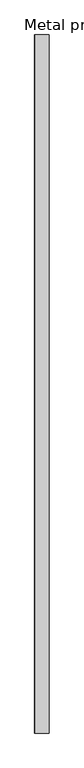
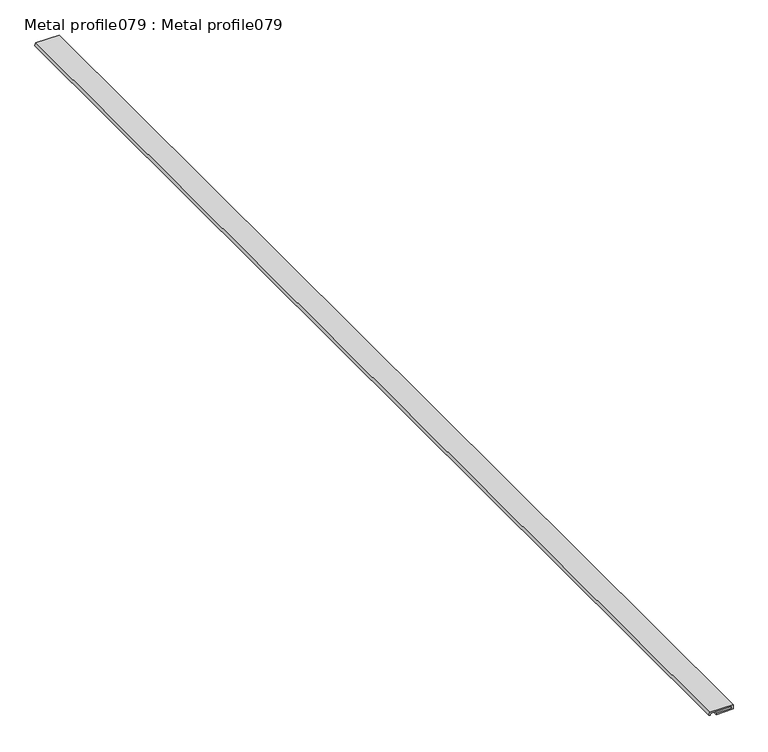
"""IFC4 building model written with IfcOpenShell, lengths in millimetres: proxy geometry, Metal profile079 : Metal profile079."""

from ifc_helpers import new_model, si_unit, frame, origin, place, context, project, spatial, polyline, outline, extrude, source, transform, mapped, element, save


def metal_profile079_metal_profile079_eafd9208(model_context):
    return source(origin(), model_context, "Body", "SweptSolid", [
        extrude(outline(polyline([(40172.6132812, -9397.2722564), (40170.6132812, -9397.2722564), (40170.6132812, -9368.0046783), (40177.890625, -9368.0046783), (40178.484375, -9407.6785064), (40173.4296875, -9409.304483), (40172.8172405, -9407.4005637), (40176.4624429, -9406.227986), (40175.9203326, -9370.0046783), (40172.6132812, -9370.0046783), (40172.6132812, -9397.2722564)])), frame((0.0, 7982.1531721, 0.0), z_axis=(0.0, 1.0, 0.0), x_axis=(0.0, 0.0, 1.0)), (0.0, 0.0, 1.0), 2000.0),
    ])


if __name__ == "__main__":
    model = new_model("IFC4")
    model_context = context("Model", 3, world=origin())
    ifc_project = project(units=[si_unit("LENGTHUNIT", "METRE", prefix="MILLI")], contexts=[model_context])
    site = spatial("IfcSite", under=ifc_project)
    building = spatial("IfcBuilding", under=site)
    placement = place(None, origin())
    metal_profile079_metal_profile079_shape = metal_profile079_metal_profile079_eafd9208(model_context)
    element("IfcBuildingElementProxy", 1, Name="Metal profile079 : Metal profile079", ObjectType="Metal profile079 : Metal profile079", at=placement, inside=building, context=model_context, shape_type="MappedRepresentation", body=[
        mapped(metal_profile079_metal_profile079_shape, transform((0.0, 0.0, 0.0), x_axis=(1.0, 0.0, 0.0), y_axis=(0.0, 1.0, 0.0), z_axis=(0.0, 0.0, 1.0))),
    ])
    save(model, "model.ifc")

# Revit data of these elements
# Type "Metal profile079 : Metal profile079"
#   NameOverride = "Metal profile079"
# Element 1 (IfcBuildingElementProxy, "Metal profile079 : Metal profile079")
#   Materials on its faces: "ANGLE TRIM"
# Materials
#   "ANGLE TRIM": class "Unassigned", colour RGB 250 255 0, transparency 0
